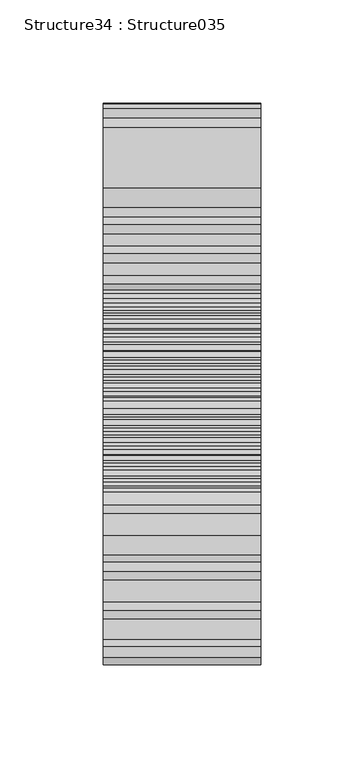
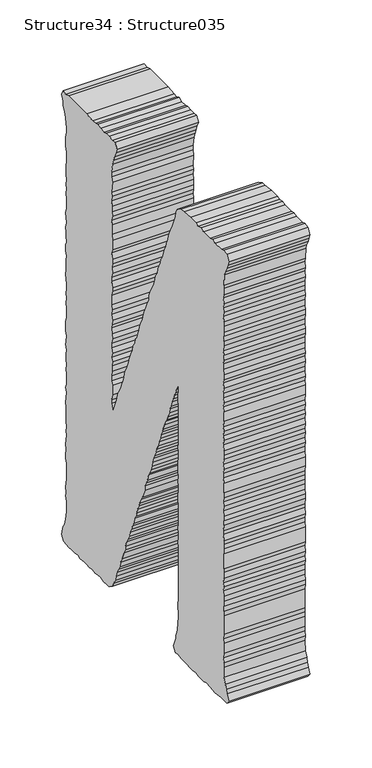
"""IFC4 building model written with IfcOpenShell, lengths in millimetres: proxy geometry, Structure34 : Structure035."""

import ifcopenshell
import ifcopenshell.guid

model = None  # the IFC model being written
_history = None  # IfcOwnerHistory: only IFC2X3 demands one
_inside = {}  # id of a spatial element -> (the spatial element, [elements in it])
_under = {}  # id of a project, library or spatial element -> (it, [spatial elements below it])
_declared = {}  # id of a project -> (the project, [libraries it declares])
_typed = {}  # id of a type object -> (the type object, [elements of that type])
_made_of = {}  # id of a material, layer set ... -> (it, [elements and type objects made of it])


def new_model(schema):
    """Start an empty IFC model of exactly this schema.

    Asked for "IFC4X3", IfcOpenShell would pick the latest addendum, in which some entities
    have other attributes; the version numbers below select the first issue.
    IFC2X3 requires an IfcOwnerHistory on every rooted entity: one is made here for all.
    """
    global model, _history
    if schema == "IFC4X3":
        model = ifcopenshell.file(schema_version=(4, 3, 0, 0))
    else:
        model = ifcopenshell.file(schema=schema)
    _inside.clear()
    _under.clear()
    _declared.clear()
    _typed.clear()
    _made_of.clear()
    _history = None
    if model.schema == "IFC2X3":
        org = make("IfcOrganization", Name="unknown")
        user = make(
            "IfcPersonAndOrganization",
            ThePerson=make("IfcPerson", FamilyName="unknown"),
            TheOrganization=org,
        )
        app = make(
            "IfcApplication",
            ApplicationDeveloper=org,
            Version="unknown",
            ApplicationFullName="unknown",
            ApplicationIdentifier="unknown",
        )
        _history = make(
            "IfcOwnerHistory",
            OwningUser=user,
            OwningApplication=app,
            ChangeAction="ADDED",
            CreationDate=0,
        )
    return model


def make(cls, **values):
    """One entity of the class cls with the attributes given. An attribute that is None is left unset."""
    return model.create_entity(
        cls, **{name: value for name, value in values.items() if value is not None}
    )


def rooted(cls, **values):
    """An entity with a GlobalId (a new one), such as an element, a storey or a relation."""
    return make(cls, GlobalId=ifcopenshell.guid.new(), OwnerHistory=_history, **values)


def si_unit(unit_type, name, prefix=None):
    """IfcSIUnit, for example si_unit("LENGTHUNIT", "METRE", prefix="MILLI")."""
    return make("IfcSIUnit", UnitType=unit_type, Prefix=prefix, Name=name)


def assignment(units):
    """IfcUnitAssignment: the units of a project."""
    return None if units is None else make("IfcUnitAssignment", Units=units)


def point(xyz):
    """IfcCartesianPoint."""
    return None if xyz is None else make("IfcCartesianPoint", Coordinates=xyz)


def direction(xyz):
    """IfcDirection."""
    return None if xyz is None else make("IfcDirection", DirectionRatios=xyz)


def frame(location, z_axis=None, x_axis=None):
    """IfcAxis2Placement3D, a coordinate frame: its origin and axes. An axis left out is left unset."""
    return make(
        "IfcAxis2Placement3D",
        Location=point(location),
        Axis=direction(z_axis),
        RefDirection=direction(x_axis),
    )


def origin():
    """The frame at (0, 0, 0) with its axes left unset."""
    return frame((0.0, 0.0, 0.0))


def place(relative_to, where):
    """IfcLocalPlacement: puts the frame where relative to a parent placement (None: the world)."""
    return make(
        "IfcLocalPlacement", PlacementRelTo=relative_to, RelativePlacement=where
    )


def context(
    kind, dimensions, precision=None, world=None, true_north=None, identifier=None
):
    """IfcGeometricRepresentationContext, for example the 3D "Model" context."""
    return make(
        "IfcGeometricRepresentationContext",
        ContextIdentifier=identifier,
        ContextType=kind,
        CoordinateSpaceDimension=dimensions,
        Precision=precision,
        WorldCoordinateSystem=world,
        TrueNorth=true_north,
    )


def project(units=None, contexts=None):
    """IfcProject with its units and contexts."""
    return rooted(
        "IfcProject",
        Name="project",
        RepresentationContexts=contexts,
        UnitsInContext=assignment(units),
    )


def spatial(cls, under=None, at=None, **own):
    """A site, building, storey or space (cls), placed at a placement, below another one or the project."""
    s = rooted(cls, ObjectPlacement=at, **own)
    if under is not None:
        _under.setdefault(under.id(), (under, []))[1].append(s)
    return s


def polyline(points):
    """IfcPolyline through the points."""
    return make("IfcPolyline", Points=[point(p) for p in points])


def outline(outer, holes=None, kind="AREA"):
    """IfcArbitraryClosedProfileDef: a profile drawn as a closed curve; with holes, ...WithVoids."""
    if holes is None:
        return make("IfcArbitraryClosedProfileDef", ProfileType=kind, OuterCurve=outer)
    return make(
        "IfcArbitraryProfileDefWithVoids",
        ProfileType=kind,
        OuterCurve=outer,
        InnerCurves=holes,
    )


def extrude(swept, where, along, depth):
    """IfcExtrudedAreaSolid: the profile swept, set in the frame where, extruded along a direction by depth."""
    return make(
        "IfcExtrudedAreaSolid",
        SweptArea=swept,
        Position=where,
        ExtrudedDirection=direction(along),
        Depth=depth,
    )


def shape(context_of_items, identifier, shape_type, items):
    """IfcShapeRepresentation: the items that make up one representation, for example the "Body"."""
    return make(
        "IfcShapeRepresentation",
        ContextOfItems=context_of_items,
        RepresentationIdentifier=identifier,
        RepresentationType=shape_type,
        Items=items,
    )


def source(mapping_origin, context_of_items, identifier, shape_type, items):
    """IfcRepresentationMap: a shape defined once, which mapped items show again and again."""
    return make(
        "IfcRepresentationMap",
        MappingOrigin=mapping_origin,
        MappedRepresentation=shape(context_of_items, identifier, shape_type, items),
    )


def transform(
    local_origin,
    x_axis=None,
    y_axis=None,
    z_axis=None,
    scale=None,
    scale2=None,
    scale3=None,
    uniform=True,
):
    """IfcCartesianTransformationOperator3D, or its non-uniform kind. x_axis, y_axis, z_axis: its Axis1, 2, 3."""
    if uniform:
        return make(
            "IfcCartesianTransformationOperator3D",
            Axis1=direction(x_axis),
            Axis2=direction(y_axis),
            LocalOrigin=point(local_origin),
            Scale=scale,
            Axis3=direction(z_axis),
        )
    return make(
        "IfcCartesianTransformationOperator3DnonUniform",
        Axis1=direction(x_axis),
        Axis2=direction(y_axis),
        LocalOrigin=point(local_origin),
        Scale=scale,
        Axis3=direction(z_axis),
        Scale2=scale2,
        Scale3=scale3,
    )


def mapped(mapping_source, mapping_target):
    """IfcMappedItem: shows the shape of a source again, moved by a transform."""
    return make(
        "IfcMappedItem", MappingSource=mapping_source, MappingTarget=mapping_target
    )


def made_of(thing, what):
    """Note that an element or type object is made of a material, layer set ...; save() writes the relation."""
    if what is not None:
        _made_of.setdefault(what.id(), (what, []))[1].append(thing)
    return thing


def element(
    cls,
    number,
    at=None,
    inside=None,
    cuts=None,
    type_object=None,
    material=None,
    context=None,
    identifier="Body",
    shape_type=None,
    held_by="IfcProductDefinitionShape",
    body=None,
    shapes=None,
    **own,
):
    """One element of the class cls, such as IfcWall. Its Tag is "e" and its number.

    at: its placement. inside: the storey or other place that contains it. cuts: it is an
    opening in that element (IfcRelVoidsElement). A single representation is given by context,
    identifier, shape_type and body (its items); several are given by shapes. held_by: the class
    of the entity that holds the representations. save() writes the other relations.
    """
    e = rooted(cls, Tag="e%d" % number, ObjectPlacement=at, **own)
    if body is not None:
        shapes = [shape(context, identifier, shape_type, body)]
    if shapes is not None:
        e.Representation = make(held_by, Representations=shapes)
    if inside is not None:
        _inside.setdefault(inside.id(), (inside, []))[1].append(e)
    if cuts is not None:
        rooted(
            "IfcRelVoidsElement", RelatingBuildingElement=cuts, RelatedOpeningElement=e
        )
    if type_object is not None:
        _typed.setdefault(type_object.id(), (type_object, []))[1].append(e)
    return made_of(e, material)


def aggregate(whole, parts):
    """IfcRelAggregates: a whole, such as a stair, and the parts it consists of."""
    return rooted("IfcRelAggregates", RelatingObject=whole, RelatedObjects=parts)


def save(model, path):
    """Write the relations noted so far, then the file.

    IfcRelAggregates (storeys below a building ...), IfcRelContainedInSpatialStructure (elements
    in a storey), IfcRelDefinesByType, IfcRelAssociatesMaterial and IfcRelDeclares: one each for
    every whole, place, type object, material and project.
    """
    for whole, parts in _under.values():
        aggregate(whole, parts)
    for where, things in _inside.values():
        rooted(
            "IfcRelContainedInSpatialStructure",
            RelatedElements=things,
            RelatingStructure=where,
        )
    for kind, things in _typed.values():
        rooted("IfcRelDefinesByType", RelatedObjects=things, RelatingType=kind)
    for what, things in _made_of.values():
        rooted("IfcRelAssociatesMaterial", RelatedObjects=things, RelatingMaterial=what)
    for by, libraries in _declared.values():
        rooted("IfcRelDeclares", RelatingContext=by, RelatedDefinitions=libraries)
    model.write(path)


def structure34_structure035_11804754(model_context):
    return source(origin(), model_context, "Body", "SweptSolid", [
        extrude(outline(polyline([(254413.231868, 3575.0851816), (254414.9921192, 3569.2524442), (254415.5713814, 3565.7094775), (254419.0918837, 3556.3417965), (254416.1731081, 3551.0658569), (254411.4700123, 3551.6675836), (254406.7909856, 3551.0658569), (254396.8279963, 3551.0658569), (254393.307494, 3550.4833855), (254388.0476005, 3550.4833855), (254383.9253715, 3551.0658569), (254378.665478, 3550.4833855), (254369.8850822, 3550.4833855), (254365.7837131, 3551.6675836), (254359.9220929, 3551.6675836), (254356.4015906, 3550.4833855), (254351.7209593, 3550.4833855), (254342.3388368, 3551.6675836), (254332.9567143, 3551.6675836), (254329.4570719, 3555.7416744), (254332.3774521, 3561.025637), (254333.558441, 3565.1254015), (254334.7169655, 3569.2524442), (254337.0564788, 3574.5107332), (254337.6582055, 3584.4689087), (254337.0564788, 3589.1527492), (254338.2374677, 3593.2541183), (254337.6582055, 3597.9540049), (254337.6582055, 3607.8961343), (254338.2374677, 3612.0135494), (254337.6582055, 3616.69739), (254337.6582055, 3635.4407751), (254337.0564788, 3640.114988), (254337.0564788, 3644.8245022), (254337.6582055, 3649.5003197), (254337.6582055, 3654.7842823), (254338.2374677, 3659.4584952), (254337.0564788, 3664.1423357), (254338.2374677, 3667.6853024), (254337.0564788, 3672.9435914), (254337.6582055, 3678.2018803), (254337.0564788, 3682.3289231), (254337.0564788, 3696.9709391), (254337.6582055, 3701.6547796), (254337.6582055, 3706.3289925), (254337.0564788, 3709.8559132), (254338.2374677, 3715.7143242), (254338.2374677, 3719.2316172), (254337.0564788, 3725.0996559), (254337.0564788, 3729.7738688), (254337.6582055, 3733.8736333), (254338.2374677, 3739.1592005), (254337.6582055, 3743.8414364), (254338.2374677, 3747.9428055), (254337.6582055, 3752.04257), (254337.0564788, 3757.3185096), (254337.0564788, 3766.684586), (254338.2374677, 3771.3860772), (254338.2374677, 3776.0618947), (254337.0564788, 3780.7441306), (254338.2374677, 3784.8438951), (254337.0564788, 3790.7039107), (254337.6582055, 3794.2292268), (254337.0564788, 3798.9050443), (254338.2374677, 3804.1890069), (254337.0564788, 3809.4729695), (254338.2374677, 3812.9726119), (254337.0564788, 3818.2309008), (254338.2374677, 3822.348316), (254337.0564788, 3828.2163546), (254337.0564788, 3837.6000817), (254338.2374677, 3841.6741725), (254337.0564788, 3846.3772683), (254338.2374677, 3851.0595042), (254338.2374677, 3855.1769193), (254337.0564788, 3861.0192843), (254338.2374677, 3865.7015202), (254337.0564788, 3869.2444869), (254337.6582055, 3873.9203044), (254338.2374677, 3879.1769888), (254338.2374677, 3884.4609514), (254337.0564788, 3888.5623205), (254337.0564788, 3893.822214), (254338.2374677, 3897.3475301), (254337.6582055, 3902.6314927), (254337.0564788, 3907.3313793), (254337.0564788, 3912.5896682), (254337.6582055, 3916.0909152), (254337.6582055, 3921.9733953), (254337.0564788, 3926.6492128), (254338.2374677, 3931.3346579), (254337.6582055, 3936.0345445), (254338.2374677, 3940.1166583), (254337.0564788, 3944.8165449), (254338.2374677, 3950.0940891), (254337.0564788, 3953.5937315), (254337.6582055, 3959.4617701), (254337.0564788, 3962.9774586), (254336.4772166, 3973.5197101), (254335.2962277, 3977.6194746), (254332.3774521, 3982.8793681), (254331.1964632, 3986.4046842), (254329.4570719, 3991.0788971), (254332.9567143, 3996.390138), (254338.2374677, 3996.9645864), (254341.7371101, 3995.7803883), (254351.7209593, 3995.7803883), (254355.8223284, 3996.9645864), (254359.9220929, 3995.7803883), (254370.4643444, 3995.7803883), (254374.5641089, 3996.9645864), (254379.2447402, 3995.7803883), (254382.7652425, 3996.9645864), (254392.1489696, 3996.9645864), (254402.6896165, 3995.7803883), (254406.7909856, 3995.7803883), (254413.231868, 3992.2614906), (254414.9921192, 3988.7634528), (254416.1731081, 3982.8793681), (254417.9108947, 3978.8036727), (254419.6711459, 3974.7055128), (254420.8537394, 3971.1785921), (254423.7949794, 3966.5043792), (254425.5327661, 3961.2204166), (254427.2930172, 3957.1190475), (254428.4756107, 3952.9920048), (254430.8151241, 3947.7337158), (254431.3943863, 3944.235678), (254433.7338997, 3939.5325823), (254435.4957554, 3934.8503464), (254437.2560065, 3930.1745289), (254439.5955199, 3926.6492128), (254440.7765088, 3922.5494483), (254442.5367599, 3917.8479571), (254444.2761512, 3914.3499193), (254445.4571401, 3909.0627475), (254448.3983802, 3904.9645876), (254449.5569046, 3900.8648231), (254450.7394981, 3895.5888836), (254453.6582737, 3890.905043), (254457.178776, 3883.2863809), (254458.9406317, 3879.1769888), (254459.5198939, 3874.5043805), (254461.8594073, 3869.8189354), (254463.6196584, 3864.5446004), (254465.9607764, 3860.4432313), (254467.1417653, 3857.5019912), (254468.9020164, 3851.6612309), (254470.0605409, 3848.7167816), (254472.4225187, 3844.0345457), (254474.1619099, 3838.7586061), (254475.3428989, 3834.6588416), (254477.10315, 3830.5574726), (254478.2616744, 3825.2911606), (254481.2045191, 3822.348316), (254481.7837813, 3817.6741031), (254484.7025569, 3813.5743386), (254485.8835458, 3808.290376), (254488.2246637, 3803.5872802), (254489.9849149, 3799.5051664), (254491.745166, 3795.4037973), (254492.3244282, 3791.8865042), (254494.6864061, 3786.0280932), (254497.027524, 3781.9299333), (254498.7877751, 3777.8285642), (254499.9462996, 3773.11905), (254501.1272885, 3768.4432325), (254502.8891442, 3764.9435901), (254504.6269309, 3760.2437036), (254506.9664443, 3755.559863), (254509.3284221, 3752.04257), (254511.66954, 3743.2332913), (254513.4297912, 3739.1592005), (254515.7693045, 3733.2991849), (254517.5311603, 3729.1737467), (254518.6896847, 3730.3563402), (254519.8706736, 3735.0578314), (254519.8706736, 3738.5574738), (254518.6896847, 3744.4158848), (254518.6896847, 3753.8012165), (254519.8706736, 3757.3185096), (254519.8706736, 3762.5848215), (254519.2914114, 3767.2590344), (254519.2914114, 3772.5606477), (254518.6896847, 3777.2444882), (254519.8706736, 3780.7441306), (254518.6896847, 3785.4456218), (254519.8706736, 3790.1294623), (254519.8706736, 3794.8309535), (254518.6896847, 3800.0876378), (254519.2914114, 3804.1890069), (254519.8706736, 3810.0474179), (254519.2914114, 3813.5743386), (254518.6896847, 3818.2309008), (254519.8706736, 3823.5341187), (254519.2914114, 3828.2163546), (254519.8706736, 3832.8921721), (254519.8706736, 3842.2758992), (254518.6896847, 3846.9757858), (254518.6896847, 3850.4754282), (254519.8706736, 3856.3161885), (254519.8706736, 3859.8591552), (254518.6896847, 3864.5446004), (254519.2914114, 3870.4030114), (254518.6896847, 3873.9203044), (254518.6896847, 3878.5784713), (254519.8706736, 3884.4609514), (254518.6896847, 3887.9621984), (254518.6896847, 3897.3475301), (254519.2914114, 3903.2059411), (254519.2914114, 3912.5896682), (254519.8706736, 3916.6653636), (254518.6896847, 3921.3748778), (254519.2914114, 3925.4746423), (254519.2914114, 3930.7329312), (254519.8706736, 3936.0345445), (254519.2914114, 3940.718385), (254519.8706736, 3944.235678), (254518.6896847, 3954.7506513), (254519.8706736, 3959.4617701), (254519.8706736, 3964.1343784), (254518.1104225, 3972.9372387), (254516.3485667, 3978.2035506), (254515.1900423, 3982.3225704), (254512.8505289, 3987.5792547), (254511.0902778, 3992.2614906), (254514.0090534, 3997.5486624), (254518.1104225, 3996.9645864), (254523.9704381, 3996.9645864), (254528.6735339, 3997.5486624), (254532.1731763, 3996.390138), (254538.0331919, 3996.390138), (254542.7138232, 3997.5486624), (254546.2343255, 3996.390138), (254550.9374213, 3996.390138), (254560.2970793, 3997.5486624), (254589.5811113, 3997.5486624), (254594.2842071, 3996.390138), (254598.9648384, 3996.9645864), (254600.7250895, 3992.2614906), (254598.9648384, 3986.4046842), (254598.3839716, 3982.8793681), (254596.0444582, 3977.6194746), (254594.2842071, 3972.9372387), (254593.1032182, 3962.9774586), (254593.1032182, 3959.4617701), (254594.2842071, 3953.5937315), (254594.2842071, 3944.8165449), (254593.1032182, 3940.1166583), (254593.1032182, 3930.1745289), (254593.7049449, 3926.6492128), (254593.7049449, 3916.6653636), (254593.1032182, 3912.0071968), (254593.7049449, 3907.3313793), (254593.1032182, 3903.2059411), (254593.7049449, 3898.5301236), (254593.1032182, 3893.246161), (254593.1032182, 3883.8881076), (254594.2842071, 3879.1769888), (254593.1032182, 3869.8189354), (254594.2842071, 3865.1190488), (254593.7049449, 3859.8591552), (254593.7049449, 3855.7353217), (254593.1032182, 3850.4754282), (254594.2842071, 3846.9757858), (254594.2842071, 3841.0900965), (254593.1032182, 3836.9919366), (254593.7049449, 3832.3161191), (254593.7049449, 3822.348316), (254594.2842071, 3818.2309008), (254593.7049449, 3812.9726119), (254593.1032182, 3809.4729695), (254593.1032182, 3804.7730829), (254593.7049449, 3799.5051664), (254593.1032182, 3795.4037973), (254593.7049449, 3790.1294623), (254593.1032182, 3784.8438951), (254593.1032182, 3775.4874463), (254594.2842071, 3771.3860772), (254594.2842071, 3762.0023501), (254593.1032182, 3757.8753073), (254593.7049449, 3752.04257), (254594.2842071, 3748.5429276), (254593.1032182, 3743.8414364), (254593.7049449, 3739.1592005), (254593.7049449, 3734.47536), (254593.1032182, 3728.5992983), (254593.7049449, 3725.0996559), (254593.1032182, 3719.2316172), (254593.1032182, 3709.8559132), (254594.2842071, 3705.7545441), (254593.1032182, 3701.6547796), (254593.7049449, 3695.786741), (254594.2842071, 3691.0868544), (254593.7049449, 3687.0127636), (254593.7049449, 3672.3691429), (254593.1032182, 3668.2437048), (254593.7049449, 3662.9854159), (254593.1032182, 3659.4584952), (254593.7049449, 3653.6000842), (254594.2842071, 3650.1004418), (254593.7049449, 3644.2420307), (254594.2842071, 3640.114988), (254594.2842071, 3635.4407751), (254593.1032182, 3631.3410106), (254593.1032182, 3616.69739), (254593.7049449, 3611.4134274), (254594.2842071, 3607.3393366), (254593.7049449, 3602.0280957), (254594.2842071, 3598.5284533), (254593.1032182, 3593.2541183), (254593.1032182, 3583.2863152), (254594.2842071, 3575.0851816), (254596.0444582, 3569.2524442), (254598.3839716, 3565.7094775), (254600.1458273, 3559.8671125), (254601.3043518, 3556.3417965), (254597.8047094, 3551.0658569), (254593.7049449, 3551.0658569), (254589.5811113, 3550.4833855), (254583.7419556, 3551.0658569), (254579.6421911, 3551.0658569), (254574.3598331, 3551.6675836), (254570.8393308, 3550.4833855), (254564.9777106, 3551.0658569), (254561.4780682, 3551.0658569), (254555.6180526, 3550.4833855), (254551.5166835, 3551.6675836), (254546.8360522, 3550.4833855), (254541.5552988, 3551.6675836), (254538.0331919, 3551.6675836), (254533.3541652, 3550.4833855), (254528.0718072, 3551.0658569), (254523.9704381, 3551.0658569), (254518.1104225, 3555.1848766), (254516.3485667, 3559.2669905), (254513.4297912, 3563.9412034), (254512.8505289, 3568.0682461), (254511.0902778, 3573.3265351), (254508.7491599, 3577.4535778), (254506.4096465, 3581.5276686), (254505.2286576, 3586.8116312), (254502.8891442, 3591.5131224), (254499.3670374, 3599.7126514), (254497.6067862, 3603.7963698), (254497.027524, 3607.3393366), (254495.2672729, 3613.1720739), (254493.5054171, 3616.69739), (254490.5866416, 3621.3732075), (254489.9849149, 3625.472972), (254487.6454015, 3630.1824862), (254485.8835458, 3634.2822506), (254483.5440324, 3638.3563415), (254482.9647702, 3643.6579547), (254480.6027924, 3647.1575971), (254478.2616744, 3651.8590883), (254477.6824122, 3655.9428067), (254475.3428989, 3660.6250426), (254474.1619099, 3664.1423357), (254472.4225187, 3668.8261762), (254469.4812786, 3672.9435914), (254465.9607764, 3681.7271964), (254465.3815141, 3686.4030139), (254463.0403962, 3691.0868544), (254461.2801451, 3694.6298211), (254460.0991561, 3700.4705815), (254458.338905, 3703.4134261), (254455.9977871, 3708.087639), (254454.2375359, 3712.7971532), (254453.6582737, 3716.8985223), (254451.8980226, 3722.1568112), (254450.1586313, 3725.6741043), (254447.7966535, 3730.3563402), (254446.6156646, 3733.8736333), (254443.696889, 3739.1592005), (254443.1176268, 3743.8414364), (254440.7765088, 3748.5429276), (254439.5955199, 3752.6170184), (254437.2560065, 3757.3185096), (254436.0750176, 3760.2437036), (254433.7338997, 3766.1021146), (254432.5753752, 3770.2018791), (254429.6341352, 3773.7015215), (254427.8947439, 3777.8285642), (254426.1344928, 3782.5027771), (254424.9535039, 3787.2042683), (254423.7949794, 3790.7039107), (254422.0122638, 3795.960595), (254419.0918837, 3800.6717138), (254417.9108947, 3804.7730829), (254416.1731081, 3808.290376), (254414.4128569, 3812.9726119), (254412.071739, 3817.6741031), (254410.8907501, 3818.2309008), (254411.4700123, 3812.9726119), (254412.071739, 3808.8888934), (254412.071739, 3803.0064134), (254411.4700123, 3798.9050443), (254410.8907501, 3794.2292268), (254411.4700123, 3790.1294623), (254411.4700123, 3780.7441306), (254410.8907501, 3774.8857196), (254410.8907501, 3766.684586), (254411.4700123, 3760.818152), (254412.071739, 3757.3185096), (254411.4700123, 3752.6170184), (254410.8907501, 3747.3587295), (254412.071739, 3742.6748889), (254412.071739, 3732.7167134), (254411.4700123, 3728.0152223), (254412.071739, 3723.9154578), (254411.4700123, 3718.6571688), (254410.8907501, 3714.5301261), (254412.071739, 3709.8559132), (254412.071739, 3704.5879966), (254411.4700123, 3700.4705815), (254410.8907501, 3696.3884676), (254410.8907501, 3691.6869765), (254411.4700123, 3687.587212), (254411.4700123, 3681.7271964), (254412.071739, 3677.0449604), (254411.4700123, 3672.3691429), (254410.8907501, 3668.2437048), (254412.071739, 3663.5598643), (254410.8907501, 3658.3015753), (254410.8907501, 3648.9258713), (254411.4700123, 3644.8245022), (254411.4700123, 3635.4407751), (254410.8907501, 3631.3410106), (254410.8907501, 3611.4134274), (254411.4700123, 3607.3393366), (254412.071739, 3602.0280957), (254412.071739, 3597.9540049), (254410.8907501, 3593.8285667), (254410.8907501, 3589.1527492), (254412.071739, 3583.2863152), (254413.231868, 3575.0851816)])), frame((-38594.2176606, 0.0, 0.0), z_axis=(1.0, 0.0, 0.0), x_axis=(0.0, 1.0, 0.0)), (0.0, 0.0, 1.0), 76.2),
    ])


if __name__ == "__main__":
    model = new_model("IFC4")
    model_context = context("Model", 3, world=origin())
    ifc_project = project(units=[si_unit("LENGTHUNIT", "METRE", prefix="MILLI")], contexts=[model_context])
    site = spatial("IfcSite", under=ifc_project)
    building = spatial("IfcBuilding", under=site)
    placement = place(None, origin())
    structure34_structure035_shape = structure34_structure035_11804754(model_context)
    element("IfcBuildingElementProxy", 1, Name="Structure34 : Structure035", ObjectType="Structure34 : Structure035", at=placement, inside=building, context=model_context, shape_type="MappedRepresentation", body=[
        mapped(structure34_structure035_shape, transform((0.0, 0.0, 0.0), x_axis=(1.0, 0.0, 0.0), y_axis=(0.0, 1.0, 0.0), z_axis=(0.0, 0.0, 1.0))),
    ])
    save(model, "model.ifc")

# Revit data of these elements
# Type "Structure34 : Structure035"
#   NameOverride = "Structure035"
# Element 1 (IfcBuildingElementProxy, "Structure34 : Structure035")
#   Materials on its faces: "BRUSHED ALUM. LETTERING"
# Materials
#   "BRUSHED ALUM. LETTERING": class "Unassigned", colour RGB 169 181 186, transparency 0, Cost = 0
